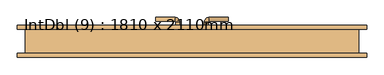
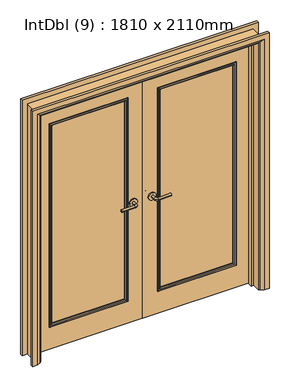
"""IFC4 building model written with IfcOpenShell, lengths in millimetres: door geometry, IntDbl (9) : 1810 x 2110mm."""

from ifc_helpers import new_model, si_unit, point, frame, frame_2d, origin, place, context, project, spatial, polyline, circle_curve, ellipse_curve, trimmed, segment, composite_curve, outline, extrude, faceted_brep, source, transform, mapped, element, save
from ifc_brep_helpers import plane_surface, cylinder_surface, revolved_surface, advanced_brep


def intdbl_9_1810_x_2110mm_150ef72f(model_context):
    return source(origin(), model_context, "Body", "SolidModel", [
        advanced_brep(
        [(-66.5, 25.0, 1007.0), (-86.5, 25.0, 1007.0), (-66.5, -5.0, 1007.0), (-86.5, -5.0, 1007.0), (-91.5, -10.0, 1007.0), (-91.5, -30.0, 1007.0), (-196.5, -30.0, 1007.0), (-196.5, -10.0, 1007.0)],
        [
            (0, 1, circle_curve(frame((-76.5, 25.0, 1007.0), z_axis=(0.0, 1.0, 0.0), x_axis=(-1.0, 0.0, 0.0)), 10.0)),
            (1, 0, circle_curve(frame((-76.5, 25.0, 1007.0), z_axis=(0.0, 1.0, 0.0), x_axis=(-1.0, 0.0, 0.0)), 10.0)),
            (0, 2),
            (2, 3, circle_curve(frame((-76.5, -5.0, 1007.0), z_axis=(0.0, 1.0, 0.0), x_axis=(-1.0, 0.0, 0.0)), 10.0)),
            (3, 1),
            (3, 2, circle_curve(frame((-76.5, -5.0, 1007.0), z_axis=(0.0, 1.0, 0.0), x_axis=(-1.0, 0.0, 0.0)), 10.0)),
            (4, 3, circle_curve(frame((-91.5, -5.0, 1007.0), z_axis=(0.0, 0.0, 1.0), x_axis=(1.0, 0.0, 0.0)), 5.0)),
            (2, 5, circle_curve(frame((-91.5, -5.0, 1007.0), z_axis=(0.0, 0.0, -1.0), x_axis=(1.0, 0.0, 0.0)), 25.0)),
            (5, 4, circle_curve(frame((-91.5, -20.0, 1007.0), z_axis=(1.0, 0.0, 0.0), x_axis=(0.0, 1.0, 0.0)), 10.0)),
            (4, 5, circle_curve(frame((-91.5, -20.0, 1007.0), z_axis=(1.0, 0.0, 0.0), x_axis=(0.0, 1.0, 0.0)), 10.0)),
            (6, 7, circle_curve(frame((-196.5, -20.0, 1007.0), z_axis=(-1.0, 0.0, 0.0), x_axis=(0.0, 1.0, 0.0)), 10.0)),
            (7, 6, circle_curve(frame((-196.5, -20.0, 1007.0), z_axis=(-1.0, 0.0, 0.0), x_axis=(0.0, 1.0, 0.0)), 10.0)),
            (5, 6),
            (7, 4),
        ],
        [
            plane_surface(frame((-76.5, 25.0, 1007.0), z_axis=(0.0, 1.0, 0.0), x_axis=(0.0, 0.0, 1.0))),
            cylinder_surface(frame((-76.5, 25.0, 1007.0), z_axis=(0.0, 1.0, 0.0), x_axis=(-1.0, 0.0, 0.0)), 10.0),
            revolved_surface(trimmed(ellipse_curve(frame((-76.5, -5.0, 1007.0), z_axis=(0.0, 1.0, 0.0), x_axis=(-1.0, 0.0, 0.0)), 10.0, 10.0), [point((-66.5, -5.0, 1007.0))], [point((-86.5, -5.0, 1007.0))], True, "CARTESIAN"), (-91.5, -5.0, 1007.0), (0.0, 0.0, -1.0)),
            revolved_surface(trimmed(ellipse_curve(frame((-76.5, -5.0, 1007.0), z_axis=(0.0, 1.0, 0.0), x_axis=(-1.0, 0.0, 0.0)), 10.0, 10.0), [point((-86.5, -5.0, 1007.0))], [point((-66.5, -5.0, 1007.0))], True, "CARTESIAN"), (-91.5, -5.0, 1007.0), (0.0, 0.0, -1.0)),
            plane_surface(frame((-196.5, -20.0, 1007.0), z_axis=(-1.0, 0.0, 0.0), x_axis=(0.0, 0.0, 1.0))),
            cylinder_surface(frame((-91.5, -20.0, 1007.0), z_axis=(1.0, 0.0, 0.0), x_axis=(0.0, 1.0, 0.0)), 10.0),
        ],
        [
            (0, [[1, 2]]),
            (1, [[-1, 3, 4, 5]]),
            (1, [[-2, -5, 6, -3]]),
            (2, [[7, -4, 8, 9]]),
            (3, [[-8, -6, -7, 10]]),
            (4, [[11, 12]]),
            (5, [[-9, 13, -12, 14]]),
            (5, [[-10, -14, -11, -13]]),
        ],
    ),
        extrude(outline(composite_curve([segment(trimmed(circle_curve(frame_2d((1007.0, -74.0)), 30.0), [point((1007.0, -44.0))], [point((1007.0, -104.0))], False, "CARTESIAN"), True, "CONTINUOUS"), segment(trimmed(circle_curve(frame_2d((1007.0, -74.0)), 30.0), [point((1007.0, -104.0))], [point((1007.0, -44.0))], False, "CARTESIAN"), True, "CONTINUOUS")], self_intersect=False)), frame((0.0, 25.0, 0.0), z_axis=(0.0, 1.0, 0.0), x_axis=(0.0, 0.0, 1.0)), (0.0, 0.0, 1.0), 8.0),
        advanced_brep(
        [(-66.5, 73.0, 1007.0), (-86.5, 73.0, 1007.0), (-86.5, 103.0, 1007.0), (-66.5, 103.0, 1007.0), (-91.5, 108.0, 1007.0), (-91.5, 128.0, 1007.0), (-196.5, 128.0, 1007.0), (-196.5, 108.0, 1007.0)],
        [
            (0, 1, circle_curve(frame((-76.5, 73.0, 1007.0), z_axis=(0.0, -1.0, 0.0), x_axis=(-1.0, 0.0, 0.0)), 10.0)),
            (1, 0, circle_curve(frame((-76.5, 73.0, 1007.0), z_axis=(0.0, -1.0, 0.0), x_axis=(-1.0, 0.0, 0.0)), 10.0)),
            (1, 2),
            (2, 3, circle_curve(frame((-76.5, 103.0, 1007.0), z_axis=(0.0, -1.0, 0.0), x_axis=(-1.0, 0.0, 0.0)), 10.0)),
            (3, 0),
            (3, 2, circle_curve(frame((-76.5, 103.0, 1007.0), z_axis=(0.0, -1.0, 0.0), x_axis=(-1.0, 0.0, 0.0)), 10.0)),
            (4, 5, circle_curve(frame((-91.5, 118.0, 1007.0), z_axis=(1.0, 0.0, 0.0), x_axis=(0.0, -1.0, 0.0)), 10.0)),
            (5, 3, circle_curve(frame((-91.5, 103.0, 1007.0), z_axis=(0.0, 0.0, -1.0), x_axis=(1.0, 0.0, 0.0)), 25.0)),
            (2, 4, circle_curve(frame((-91.5, 103.0, 1007.0), z_axis=(0.0, 0.0, 1.0), x_axis=(1.0, 0.0, 0.0)), 5.0)),
            (5, 4, circle_curve(frame((-91.5, 118.0, 1007.0), z_axis=(1.0, 0.0, 0.0), x_axis=(0.0, -1.0, 0.0)), 10.0)),
            (6, 7, circle_curve(frame((-196.5, 118.0, 1007.0), z_axis=(-1.0, 0.0, 0.0), x_axis=(0.0, -1.0, 0.0)), 10.0)),
            (7, 6, circle_curve(frame((-196.5, 118.0, 1007.0), z_axis=(-1.0, 0.0, 0.0), x_axis=(0.0, -1.0, 0.0)), 10.0)),
            (4, 7),
            (6, 5),
        ],
        [
            plane_surface(frame((-76.5, 73.0, 1007.0), z_axis=(0.0, -1.0, 0.0), x_axis=(0.0, 0.0, 1.0))),
            cylinder_surface(frame((-76.5, 73.0, 1007.0), z_axis=(0.0, -1.0, 0.0), x_axis=(-1.0, 0.0, 0.0)), 10.0),
            revolved_surface(trimmed(ellipse_curve(frame((-76.5, 103.0, 1007.0), z_axis=(0.0, 1.0, 0.0), x_axis=(-1.0, 0.0, 0.0)), 10.0, 10.0), [point((-66.5, 103.0, 1007.0))], [point((-86.5, 103.0, 1007.0))], True, "CARTESIAN"), (-91.5, 103.0, 1007.0), (0.0, 0.0, -1.0)),
            revolved_surface(trimmed(ellipse_curve(frame((-76.5, 103.0, 1007.0), z_axis=(0.0, 1.0, 0.0), x_axis=(-1.0, 0.0, 0.0)), 10.0, 10.0), [point((-86.5, 103.0, 1007.0))], [point((-66.5, 103.0, 1007.0))], True, "CARTESIAN"), (-91.5, 103.0, 1007.0), (0.0, 0.0, -1.0)),
            plane_surface(frame((-196.5, 118.0, 1007.0), z_axis=(-1.0, 0.0, 0.0), x_axis=(0.0, 0.0, 1.0))),
            cylinder_surface(frame((-91.5, 118.0, 1007.0), z_axis=(1.0, 0.0, 0.0), x_axis=(0.0, -1.0, 0.0)), 10.0),
        ],
        [
            (0, [[1, 2]]),
            (1, [[3, 4, 5, -2]]),
            (1, [[-5, 6, -3, -1]]),
            (2, [[7, 8, -4, 9]]),
            (3, [[10, -9, -6, -8]]),
            (4, [[11, 12]]),
            (5, [[13, -11, 14, -7]]),
            (5, [[-14, -12, -13, -10]]),
        ],
    ),
        extrude(outline(composite_curve([segment(trimmed(circle_curve(frame_2d((1007.0, -74.0)), 30.0), [point((1007.0, -44.0))], [point((1007.0, -104.0))], False, "CARTESIAN"), True, "CONTINUOUS"), segment(trimmed(circle_curve(frame_2d((1007.0, -74.0)), 30.0), [point((1007.0, -104.0))], [point((1007.0, -44.0))], False, "CARTESIAN"), True, "CONTINUOUS")], self_intersect=False)), frame((0.0, 65.0, 0.0), z_axis=(0.0, 1.0, 0.0), x_axis=(0.0, 0.0, 1.0)), (0.0, 0.0, 1.0), 8.0),
        advanced_brep(
        [(66.5, 25.0, 1007.0), (86.5, 25.0, 1007.0), (86.5, -5.0, 1007.0), (66.5, -5.0, 1007.0), (91.5, -10.0, 1007.0), (91.5, -30.0, 1007.0), (196.5, -30.0, 1007.0), (196.5, -10.0, 1007.0)],
        [
            (0, 1, circle_curve(frame((76.5, 25.0, 1007.0), z_axis=(0.0, 1.0, 0.0), x_axis=(1.0, 0.0, 0.0)), 10.0)),
            (1, 0, circle_curve(frame((76.5, 25.0, 1007.0), z_axis=(0.0, 1.0, 0.0), x_axis=(1.0, 0.0, 0.0)), 10.0)),
            (1, 2),
            (2, 3, circle_curve(frame((76.5, -5.0, 1007.0), z_axis=(0.0, 1.0, 0.0), x_axis=(1.0, 0.0, 0.0)), 10.0)),
            (3, 0),
            (3, 2, circle_curve(frame((76.5, -5.0, 1007.0), z_axis=(0.0, 1.0, 0.0), x_axis=(1.0, 0.0, 0.0)), 10.0)),
            (4, 5, circle_curve(frame((91.5, -20.0, 1007.0), z_axis=(-1.0, 0.0, 0.0), x_axis=(0.0, 1.0, 0.0)), 10.0)),
            (5, 3, circle_curve(frame((91.5, -5.0, 1007.0), z_axis=(0.0, 0.0, -1.0), x_axis=(-1.0, 0.0, 0.0)), 25.0)),
            (2, 4, circle_curve(frame((91.5, -5.0, 1007.0), z_axis=(0.0, 0.0, 1.0), x_axis=(-1.0, 0.0, 0.0)), 5.0)),
            (5, 4, circle_curve(frame((91.5, -20.0, 1007.0), z_axis=(-1.0, 0.0, 0.0), x_axis=(0.0, 1.0, 0.0)), 10.0)),
            (6, 7, circle_curve(frame((196.5, -20.0, 1007.0), z_axis=(1.0, 0.0, 0.0), x_axis=(0.0, 1.0, 0.0)), 10.0)),
            (7, 6, circle_curve(frame((196.5, -20.0, 1007.0), z_axis=(1.0, 0.0, 0.0), x_axis=(0.0, 1.0, 0.0)), 10.0)),
            (4, 7),
            (6, 5),
        ],
        [
            plane_surface(frame((76.5, 25.0, 1007.0), z_axis=(0.0, 1.0, 0.0), x_axis=(0.0, 0.0, 1.0))),
            cylinder_surface(frame((76.5, 25.0, 1007.0), z_axis=(0.0, 1.0, 0.0), x_axis=(1.0, 0.0, 0.0)), 10.0),
            revolved_surface(trimmed(ellipse_curve(frame((76.5, -5.0, 1007.0), z_axis=(0.0, -1.0, 0.0), x_axis=(1.0, 0.0, 0.0)), 10.0, 10.0), [point((66.5, -5.0, 1007.0))], [point((86.5, -5.0, 1007.0))], True, "CARTESIAN"), (91.5, -5.0, 1007.0), (0.0, 0.0, -1.0)),
            revolved_surface(trimmed(ellipse_curve(frame((76.5, -5.0, 1007.0), z_axis=(0.0, -1.0, 0.0), x_axis=(1.0, 0.0, 0.0)), 10.0, 10.0), [point((86.5, -5.0, 1007.0))], [point((66.5, -5.0, 1007.0))], True, "CARTESIAN"), (91.5, -5.0, 1007.0), (0.0, 0.0, -1.0)),
            plane_surface(frame((196.5, -20.0, 1007.0), z_axis=(1.0, 0.0, 0.0), x_axis=(0.0, 0.0, 1.0))),
            cylinder_surface(frame((91.5, -20.0, 1007.0), z_axis=(-1.0, 0.0, 0.0), x_axis=(0.0, 1.0, 0.0)), 10.0),
        ],
        [
            (0, [[1, 2]]),
            (1, [[3, 4, 5, -2]]),
            (1, [[-5, 6, -3, -1]]),
            (2, [[7, 8, -4, 9]]),
            (3, [[10, -9, -6, -8]]),
            (4, [[11, 12]]),
            (5, [[13, -11, 14, -7]]),
            (5, [[-14, -12, -13, -10]]),
        ],
    ),
        extrude(outline(composite_curve([segment(trimmed(circle_curve(frame_2d((1007.0, 74.0)), 30.0), [point((1007.0, 44.0))], [point((1007.0, 104.0))], False, "CARTESIAN"), True, "CONTINUOUS"), segment(trimmed(circle_curve(frame_2d((1007.0, 74.0)), 30.0), [point((1007.0, 104.0))], [point((1007.0, 44.0))], False, "CARTESIAN"), True, "CONTINUOUS")], self_intersect=False)), frame((0.0, 25.0, 0.0), z_axis=(0.0, 1.0, 0.0), x_axis=(0.0, 0.0, 1.0)), (0.0, 0.0, 1.0), 8.0),
        advanced_brep(
        [(66.5, 73.0, 1007.0), (86.5, 73.0, 1007.0), (66.5, 103.0, 1007.0), (86.5, 103.0, 1007.0), (91.5, 108.0, 1007.0), (91.5, 128.0, 1007.0), (196.5, 128.0, 1007.0), (196.5, 108.0, 1007.0)],
        [
            (0, 1, circle_curve(frame((76.5, 73.0, 1007.0), z_axis=(0.0, -1.0, 0.0), x_axis=(1.0, 0.0, 0.0)), 10.0)),
            (1, 0, circle_curve(frame((76.5, 73.0, 1007.0), z_axis=(0.0, -1.0, 0.0), x_axis=(1.0, 0.0, 0.0)), 10.0)),
            (0, 2),
            (2, 3, circle_curve(frame((76.5, 103.0, 1007.0), z_axis=(0.0, -1.0, 0.0), x_axis=(1.0, 0.0, 0.0)), 10.0)),
            (3, 1),
            (3, 2, circle_curve(frame((76.5, 103.0, 1007.0), z_axis=(0.0, -1.0, 0.0), x_axis=(1.0, 0.0, 0.0)), 10.0)),
            (4, 3, circle_curve(frame((91.5, 103.0, 1007.0), z_axis=(0.0, 0.0, 1.0), x_axis=(-1.0, 0.0, 0.0)), 5.0)),
            (2, 5, circle_curve(frame((91.5, 103.0, 1007.0), z_axis=(0.0, 0.0, -1.0), x_axis=(-1.0, 0.0, 0.0)), 25.0)),
            (5, 4, circle_curve(frame((91.5, 118.0, 1007.0), z_axis=(-1.0, 0.0, 0.0), x_axis=(0.0, -1.0, 0.0)), 10.0)),
            (4, 5, circle_curve(frame((91.5, 118.0, 1007.0), z_axis=(-1.0, 0.0, 0.0), x_axis=(0.0, -1.0, 0.0)), 10.0)),
            (6, 7, circle_curve(frame((196.5, 118.0, 1007.0), z_axis=(1.0, 0.0, 0.0), x_axis=(0.0, -1.0, 0.0)), 10.0)),
            (7, 6, circle_curve(frame((196.5, 118.0, 1007.0), z_axis=(1.0, 0.0, 0.0), x_axis=(0.0, -1.0, 0.0)), 10.0)),
            (5, 6),
            (7, 4),
        ],
        [
            plane_surface(frame((76.5, 73.0, 1007.0), z_axis=(0.0, -1.0, 0.0), x_axis=(0.0, 0.0, 1.0))),
            cylinder_surface(frame((76.5, 73.0, 1007.0), z_axis=(0.0, -1.0, 0.0), x_axis=(1.0, 0.0, 0.0)), 10.0),
            revolved_surface(trimmed(ellipse_curve(frame((76.5, 103.0, 1007.0), z_axis=(0.0, -1.0, 0.0), x_axis=(1.0, 0.0, 0.0)), 10.0, 10.0), [point((66.5, 103.0, 1007.0))], [point((86.5, 103.0, 1007.0))], True, "CARTESIAN"), (91.5, 103.0, 1007.0), (0.0, 0.0, -1.0)),
            revolved_surface(trimmed(ellipse_curve(frame((76.5, 103.0, 1007.0), z_axis=(0.0, -1.0, 0.0), x_axis=(1.0, 0.0, 0.0)), 10.0, 10.0), [point((86.5, 103.0, 1007.0))], [point((66.5, 103.0, 1007.0))], True, "CARTESIAN"), (91.5, 103.0, 1007.0), (0.0, 0.0, -1.0)),
            plane_surface(frame((196.5, 118.0, 1007.0), z_axis=(1.0, 0.0, 0.0), x_axis=(0.0, 0.0, 1.0))),
            cylinder_surface(frame((91.5, 118.0, 1007.0), z_axis=(-1.0, 0.0, 0.0), x_axis=(0.0, -1.0, 0.0)), 10.0),
        ],
        [
            (0, [[1, 2]]),
            (1, [[-1, 3, 4, 5]]),
            (1, [[-2, -5, 6, -3]]),
            (2, [[7, -4, 8, 9]]),
            (3, [[-8, -6, -7, 10]]),
            (4, [[11, 12]]),
            (5, [[-9, 13, -12, 14]]),
            (5, [[-10, -14, -11, -13]]),
        ],
    ),
        extrude(outline(composite_curve([segment(trimmed(circle_curve(frame_2d((1007.0, 74.0)), 30.0), [point((1007.0, 44.0))], [point((1007.0, 104.0))], False, "CARTESIAN"), True, "CONTINUOUS"), segment(trimmed(circle_curve(frame_2d((1007.0, 74.0)), 30.0), [point((1007.0, 104.0))], [point((1007.0, 44.0))], False, "CARTESIAN"), True, "CONTINUOUS")], self_intersect=False)), frame((0.0, 65.0, 0.0), z_axis=(0.0, 1.0, 0.0), x_axis=(0.0, 0.0, 1.0)), (0.0, 0.0, 1.0), 8.0),
        advanced_brep(
        [(-940.0, -85.0, 0.0), (-940.0, -65.0, 0.0), (-870.0, -65.0, 0.0), (-874.0, -71.0, 0.0), (-900.0, -85.0, 0.0), (-940.0, -85.0, 2145.0), (-940.0, -65.0, 2145.0), (940.0, -65.0, 2145.0), (940.0, -65.0, 0.0), (870.0, -65.0, 0.0), (870.0, -65.0, 2075.0), (-870.0, -65.0, 2075.0), (-874.0, -71.0, 2079.0), (-900.0, -85.0, 2105.0), (900.0, -85.0, 2105.0), (900.0, -85.0, 0.0), (940.0, -85.0, 0.0), (940.0, -85.0, 2145.0), (874.0, -71.0, 0.0), (874.0, -71.0, 2079.0)],
        [
            (0, 1),
            (1, 2),
            (2, 3, circle_curve(frame((-878.0, -64.0, 0.0), z_axis=(0.0, 0.0, -1.0), x_axis=(-1.0, 0.0, 0.0)), 8.0622577)),
            (3, 4),
            (4, 0),
            (0, 5),
            (5, 6),
            (6, 1),
            (6, 7),
            (7, 8),
            (8, 9),
            (9, 10),
            (10, 11),
            (11, 2),
            (11, 12, ellipse_curve(frame((-878.0, -64.0, 2083.0), z_axis=(-0.7071067811865475, 0.0, -0.7071067811865475), x_axis=(0.7071067811865474, 0.0, -0.7071067811865476)), 11.4017543, 8.0622577)),
            (12, 3),
            (12, 13),
            (13, 4),
            (13, 14),
            (14, 15),
            (15, 16),
            (16, 17),
            (17, 5),
            (7, 17),
            (16, 8),
            (15, 18),
            (18, 9, circle_curve(frame((878.0, -64.0, 0.0), z_axis=(0.0, 0.0, -1.0), x_axis=(1.0, 0.0, 0.0)), 8.0622577)),
            (19, 10, ellipse_curve(frame((878.0, -64.0, 2083.0), z_axis=(0.7071067811865475, 0.0, -0.7071067811865475), x_axis=(0.7071067811865474, 0.0, 0.7071067811865476)), 11.4017543, 8.0622577)),
            (18, 19),
            (14, 19),
            (19, 12),
        ],
        [
            plane_surface(frame((-870.0, -65.0, 0.0), z_axis=(0.0, 0.0, -1.0), x_axis=(0.0, -1.0, 0.0))),
            plane_surface(frame((-940.0, -85.0, 0.0), z_axis=(-1.0, 0.0, 0.0), x_axis=(0.0, 0.0, 1.0))),
            plane_surface(frame((-940.0, -65.0, 0.0), z_axis=(0.0, 1.0, 0.0), x_axis=(0.0, 0.0, 1.0))),
            cylinder_surface(frame((-878.0, -64.0, 0.0), z_axis=(0.0, 0.0, -1.0), x_axis=(-1.0, 0.0, 0.0)), 8.0622577),
            plane_surface(frame((-874.0, -71.0, 0.0), z_axis=(0.4740998230350183, -0.8804710999221749, 0.0), x_axis=(0.0, 0.0, 1.0))),
            plane_surface(frame((-900.0, -85.0, 0.0), z_axis=(0.0, -1.0, 0.0), x_axis=(0.0, 0.0, 1.0))),
            plane_surface(frame((940.0, -85.0, 2145.0), z_axis=(1.0, 0.0, 0.0), x_axis=(0.0, 0.0, -1.0))),
            plane_surface(frame((870.0, -65.0, 0.0), z_axis=(0.0, 0.0, -1.0), x_axis=(0.0, -1.0, 0.0))),
            cylinder_surface(frame((878.0, -64.0, 2075.0), z_axis=(0.0, 0.0, 1.0), x_axis=(1.0, 0.0, 0.0)), 8.0622577),
            plane_surface(frame((874.0, -71.0, 2079.0), z_axis=(-0.4740998230350183, -0.8804710999221749, 0.0), x_axis=(0.0, 0.0, -1.0))),
            plane_surface(frame((-940.0, -85.0, 2145.0), z_axis=(0.0, 0.0, 1.0), x_axis=(1.0, 0.0, 0.0))),
            cylinder_surface(frame((-870.0, -64.0, 2083.0), z_axis=(-1.0, 0.0, 0.0), x_axis=(0.0, 0.0, 1.0)), 8.0622577),
            plane_surface(frame((-874.0, -71.0, 2079.0), z_axis=(0.0, -0.8804710999221749, -0.4740998230350183), x_axis=(1.0, 0.0, 0.0))),
        ],
        [
            (0, [[1, 2, 3, 4, 5]]),
            (1, [[-1, 6, 7, 8]]),
            (2, [[-2, -8, 9, 10, 11, 12, 13, 14]]),
            (3, [[-3, -14, 15, 16]]),
            (4, [[-4, -16, 17, 18]]),
            (5, [[-5, -18, 19, 20, 21, 22, 23, -6]]),
            (6, [[24, -22, 25, -10]]),
            (7, [[-21, 26, 27, -11, -25]]),
            (8, [[28, -12, -27, 29]]),
            (9, [[30, -29, -26, -20]]),
            (10, [[-7, -23, -24, -9]]),
            (11, [[-15, -13, -28, 31]]),
            (12, [[-17, -31, -30, -19]]),
        ],
    ),
        advanced_brep(
        [(940.0, 85.0, 0.0), (940.0, 65.0, 0.0), (870.0, 65.0, 0.0), (874.0, 71.0, 0.0), (900.0, 85.0, 0.0), (940.0, 85.0, 2145.0), (940.0, 65.0, 2145.0), (-940.0, 65.0, 2145.0), (-940.0, 65.0, 0.0), (-870.0, 65.0, 0.0), (-870.0, 65.0, 2075.0), (870.0, 65.0, 2075.0), (874.0, 71.0, 2079.0), (900.0, 85.0, 2105.0), (-900.0, 85.0, 2105.0), (-900.0, 85.0, 0.0), (-940.0, 85.0, 0.0), (-940.0, 85.0, 2145.0), (-874.0, 71.0, 0.0), (-874.0, 71.0, 2079.0)],
        [
            (0, 1),
            (1, 2),
            (2, 3, circle_curve(frame((878.0, 64.0, 0.0), z_axis=(0.0, 0.0, -1.0), x_axis=(1.0, 0.0, 0.0)), 8.0622577)),
            (3, 4),
            (4, 0),
            (0, 5),
            (5, 6),
            (6, 1),
            (6, 7),
            (7, 8),
            (8, 9),
            (9, 10),
            (10, 11),
            (11, 2),
            (11, 12, ellipse_curve(frame((878.0, 64.0, 2083.0), z_axis=(0.7071067811865475, 0.0, -0.7071067811865475), x_axis=(-0.7071067811865474, 0.0, -0.7071067811865476)), 11.4017543, 8.0622577)),
            (12, 3),
            (12, 13),
            (13, 4),
            (13, 14),
            (14, 15),
            (15, 16),
            (16, 17),
            (17, 5),
            (7, 17),
            (16, 8),
            (15, 18),
            (18, 9, circle_curve(frame((-878.0, 64.0, 0.0), z_axis=(0.0, 0.0, -1.0), x_axis=(-1.0, 0.0, 0.0)), 8.0622577)),
            (19, 10, ellipse_curve(frame((-878.0, 64.0, 2083.0), z_axis=(-0.7071067811865475, 0.0, -0.7071067811865475), x_axis=(-0.7071067811865474, 0.0, 0.7071067811865476)), 11.4017543, 8.0622577)),
            (18, 19),
            (14, 19),
            (19, 12),
        ],
        [
            plane_surface(frame((870.0, 65.0, 0.0), z_axis=(0.0, 0.0, -1.0), x_axis=(0.0, -1.0, 0.0))),
            plane_surface(frame((940.0, 85.0, 0.0), z_axis=(1.0, 0.0, 0.0), x_axis=(0.0, 0.0, 1.0))),
            plane_surface(frame((940.0, 65.0, 0.0), z_axis=(0.0, -1.0, 0.0), x_axis=(0.0, 0.0, 1.0))),
            cylinder_surface(frame((878.0, 64.0, 0.0), z_axis=(0.0, 0.0, -1.0), x_axis=(1.0, 0.0, 0.0)), 8.0622577),
            plane_surface(frame((874.0, 71.0, 0.0), z_axis=(-0.4740998230350126, 0.8804710999221779, 0.0), x_axis=(0.0, 0.0, 1.0))),
            plane_surface(frame((900.0, 85.0, 0.0), z_axis=(0.0, 1.0, 0.0), x_axis=(0.0, 0.0, 1.0))),
            plane_surface(frame((-940.0, 85.0, 2145.0), z_axis=(-1.0, 0.0, 0.0), x_axis=(0.0, 0.0, -1.0))),
            plane_surface(frame((-870.0, 65.0, 0.0), z_axis=(0.0, 0.0, -1.0), x_axis=(0.0, -1.0, 0.0))),
            cylinder_surface(frame((-878.0, 64.0, 2075.0), z_axis=(0.0, 0.0, 1.0), x_axis=(-1.0, 0.0, 0.0)), 8.0622577),
            plane_surface(frame((-874.0, 71.0, 2079.0), z_axis=(0.4740998230350183, 0.8804710999221749, 0.0), x_axis=(0.0, 0.0, -1.0))),
            plane_surface(frame((940.0, 85.0, 2145.0), z_axis=(0.0, 0.0, 1.0), x_axis=(-1.0, 0.0, 0.0))),
            cylinder_surface(frame((870.0, 64.0, 2083.0), z_axis=(1.0, 0.0, 0.0), x_axis=(0.0, 0.0, 1.0)), 8.0622577),
            plane_surface(frame((874.0, 71.0, 2079.0), z_axis=(0.0, 0.8804710999221763, -0.4740998230350154), x_axis=(-1.0, 0.0, 0.0))),
        ],
        [
            (0, [[1, 2, 3, 4, 5]]),
            (1, [[-1, 6, 7, 8]]),
            (2, [[-2, -8, 9, 10, 11, 12, 13, 14]]),
            (3, [[-3, -14, 15, 16]]),
            (4, [[-4, -16, 17, 18]]),
            (5, [[-5, -18, 19, 20, 21, 22, 23, -6]]),
            (6, [[24, -22, 25, -10]]),
            (7, [[-21, 26, 27, -11, -25]]),
            (8, [[28, -12, -27, 29]]),
            (9, [[30, -29, -26, -20]]),
            (10, [[-7, -23, -24, -9]]),
            (11, [[-15, -13, -28, 31]]),
            (12, [[-17, -31, -30, -19]]),
        ],
    ),
        faceted_brep([(-846.0, 30.0, 0.0), (-846.0, -2.0, 0.0), (-865.0, -2.0, 0.0), (-865.0, 30.0, 0.0), (-846.0, 30.0, 2051.0), (-846.0, -2.0, 2051.0), (-865.0, -2.0, 2070.0), (-865.0, 30.0, 2070.0), (846.0, 30.0, 0.0), (865.0, 30.0, 0.0), (865.0, -2.0, 0.0), (846.0, -2.0, 0.0), (846.0, 30.0, 2051.0), (865.0, 30.0, 2070.0), (865.0, -2.0, 2070.0), (846.0, -2.0, 2051.0)], [[[0, 1, 2, 3]], [[1, 0, 4, 5]], [[2, 1, 5, 6]], [[3, 2, 6, 7]], [[0, 3, 7, 4]], [[8, 9, 10, 11]], [[12, 13, 9, 8]], [[13, 14, 10, 9]], [[14, 15, 11, 10]], [[15, 12, 8, 11]], [[5, 4, 12, 15]], [[6, 5, 15, 14]], [[7, 6, 14, 13]], [[4, 7, 13, 12]]]),
        extrude(outline(polyline([(2102.0, -897.0), (0.0, -897.0), (0.0, -865.0), (2070.0, -865.0), (2070.0, 865.0), (0.0, 865.0), (0.0, 897.0), (2102.0, 897.0), (2102.0, -897.0)])), frame((0.0, -65.0, 0.0), z_axis=(0.0, 1.0, 0.0), x_axis=(0.0, 0.0, 1.0)), (0.0, 0.0, 1.0), 130.0),
        extrude(outline(polyline([(-126.5, 43.0), (-737.0, 43.0), (-737.0, 55.0), (-126.5, 55.0), (-126.5, 43.0)])), frame((0.0, 0.0, 200.0), z_axis=(0.0, 0.0, 1.0), x_axis=(1.0, 0.0, 0.0)), (0.0, 0.0, 1.0), 1692.0),
        extrude(outline(polyline([(737.0, 43.0), (126.5, 43.0), (126.5, 55.0), (737.0, 55.0), (737.0, 43.0)])), frame((0.0, 0.0, 200.0), z_axis=(0.0, 0.0, 1.0), x_axis=(1.0, 0.0, 0.0)), (0.0, 0.0, 1.0), 1692.0),
        extrude(outline(polyline([(5.753223, -862.0), (5.753223, -1.5), (2067.0, -1.5), (2067.0, -862.0), (5.753223, -862.0)]), holes=[polyline([(1892.0, -737.0), (1892.0, -126.5), (200.0, -126.5), (200.0, -737.0), (1892.0, -737.0)])]), frame((0.0, 33.0, 0.0), z_axis=(0.0, 1.0, 0.0), x_axis=(0.0, 0.0, 1.0)), (0.0, 0.0, 1.0), 32.0),
        extrude(outline(polyline([(5.753223, 862.0), (2067.0, 862.0), (2067.0, 1.5), (5.753223, 1.5), (5.753223, 862.0)]), holes=[polyline([(1892.0, 126.5), (1892.0, 737.0), (200.0, 737.0), (200.0, 126.5), (1892.0, 126.5)])]), frame((0.0, 33.0, 0.0), z_axis=(0.0, 1.0, 0.0), x_axis=(0.0, 0.0, 1.0)), (0.0, 0.0, 1.0), 32.0),
        advanced_brep(
        [(-737.0, 55.0, 1892.0), (-737.0, 65.0, 1892.0), (-737.0, 65.0, 200.0), (-737.0, 55.0, 200.0), (-725.0, 66.0, 1880.0), (-725.0, 55.0, 1880.0), (-725.0, 55.0, 212.0), (-725.0, 66.0, 212.0), (-730.0, 71.0, 1885.0), (-730.0, 71.0, 207.0), (-745.0, 69.0, 1900.0), (-743.0, 71.0, 1898.0), (-743.0, 71.0, 194.0), (-745.0, 69.0, 192.0), (-745.0, 65.0, 1900.0), (-745.0, 65.0, 192.0), (-126.5, 65.0, 200.0), (-126.5, 55.0, 200.0), (-138.5, 55.0, 212.0), (-138.5, 66.0, 212.0), (-133.5, 71.0, 207.0), (-120.5, 71.0, 194.0), (-118.5, 69.0, 192.0), (-118.5, 65.0, 192.0), (-126.5, 65.0, 1892.0), (-126.5, 55.0, 1892.0), (-138.5, 55.0, 1880.0), (-138.5, 66.0, 1880.0), (-133.5, 71.0, 1885.0), (-120.5, 71.0, 1898.0), (-118.5, 69.0, 1900.0), (-118.5, 65.0, 1900.0)],
        [
            (0, 1),
            (1, 2),
            (2, 3),
            (3, 0),
            (4, 5),
            (5, 6),
            (6, 7),
            (7, 4),
            (8, 4, ellipse_curve(frame((-730.0, 66.0, 1885.0), z_axis=(-0.7071067811865475, 0.0, -0.7071067811865475), x_axis=(-0.7071067811865474, 0.0, 0.7071067811865476)), 7.0710678, 5.0)),
            (7, 9, ellipse_curve(frame((-730.0, 66.0, 207.0), z_axis=(-0.7071067811865475, 0.0, 0.7071067811865475), x_axis=(0.7071067811865474, 0.0, 0.7071067811865476)), 7.0710678, 5.0)),
            (9, 8),
            (10, 11, ellipse_curve(frame((-743.0, 69.0, 1898.0), z_axis=(-0.7071067811865475, 0.0, -0.7071067811865475), x_axis=(-0.7071067811865474, 0.0, 0.7071067811865476)), 2.8284271, 2.0)),
            (11, 12),
            (12, 13, ellipse_curve(frame((-743.0, 69.0, 194.0), z_axis=(-0.7071067811865475, 0.0, 0.7071067811865475), x_axis=(0.7071067811865474, 0.0, 0.7071067811865476)), 2.8284271, 2.0)),
            (13, 10),
            (14, 10),
            (13, 15),
            (15, 14),
            (2, 16),
            (16, 17),
            (17, 3),
            (6, 18),
            (18, 19),
            (19, 7),
            (19, 20, ellipse_curve(frame((-133.5, 66.0, 207.0), z_axis=(-0.7071067811865475, 0.0, -0.7071067811865475), x_axis=(-0.7071067811865476, 0.0, 0.7071067811865474)), 7.0710678, 5.0)),
            (20, 9),
            (12, 21),
            (21, 22, ellipse_curve(frame((-120.5, 69.0, 194.0), z_axis=(-0.7071067811865475, 0.0, -0.7071067811865475), x_axis=(-0.7071067811865476, 0.0, 0.7071067811865474)), 2.8284271, 2.0)),
            (22, 13),
            (22, 23),
            (23, 15),
            (16, 24),
            (24, 25),
            (25, 17),
            (18, 26),
            (26, 27),
            (27, 19),
            (27, 28, ellipse_curve(frame((-133.5, 66.0, 1885.0), z_axis=(0.7071067811865475, 0.0, -0.7071067811865475), x_axis=(-0.7071067811865474, 0.0, -0.7071067811865476)), 7.0710678, 5.0)),
            (28, 20),
            (21, 29),
            (29, 30, ellipse_curve(frame((-120.5, 69.0, 1898.0), z_axis=(0.7071067811865475, 0.0, -0.7071067811865475), x_axis=(-0.7071067811865474, 0.0, -0.7071067811865476)), 2.8284271, 2.0)),
            (30, 22),
            (30, 31),
            (31, 23),
            (31, 14),
            (1, 24),
            (0, 25),
            (5, 26),
            (4, 27),
            (8, 28),
            (11, 29),
            (10, 30),
        ],
        [
            plane_surface(frame((-737.0, 65.0, 1892.0), z_axis=(-1.0, 0.0, 0.0), x_axis=(0.0, 0.0, -1.0))),
            plane_surface(frame((-725.0, 55.0, 1880.0), z_axis=(1.0, 0.0, 0.0), x_axis=(0.0, 0.0, -1.0))),
            cylinder_surface(frame((-730.0, 66.0, 1892.0), z_axis=(0.0, 0.0, 1.0), x_axis=(-1.0, 0.0, 0.0)), 5.0),
            cylinder_surface(frame((-743.0, 69.0, 1892.0), z_axis=(0.0, 0.0, 1.0), x_axis=(-1.0, 0.0, 0.0)), 2.0),
            plane_surface(frame((-745.0, 69.0, 1900.0), z_axis=(-1.0, 0.0, 0.0), x_axis=(0.0, 0.0, -1.0))),
            plane_surface(frame((-737.0, 65.0, 200.0), z_axis=(0.0, 0.0, -1.0), x_axis=(1.0, 0.0, 0.0))),
            plane_surface(frame((-725.0, 55.0, 212.0), z_axis=(0.0, 0.0, 1.0), x_axis=(1.0, 0.0, 0.0))),
            cylinder_surface(frame((-737.0, 66.0, 207.0), z_axis=(-1.0, 0.0, 0.0), x_axis=(0.0, 0.0, -1.0)), 5.0),
            cylinder_surface(frame((-737.0, 69.0, 194.0), z_axis=(-1.0, 0.0, 0.0), x_axis=(0.0, 0.0, -1.0)), 2.0),
            plane_surface(frame((-745.0, 69.0, 192.0), z_axis=(0.0, 0.0, -1.0), x_axis=(1.0, 0.0, 0.0))),
            plane_surface(frame((-126.5, 65.0, 200.0), z_axis=(1.0, 0.0, 0.0), x_axis=(0.0, 0.0, 1.0))),
            plane_surface(frame((-138.5, 55.0, 212.0), z_axis=(-1.0, 0.0, 0.0), x_axis=(0.0, 0.0, 1.0))),
            cylinder_surface(frame((-133.5, 66.0, 200.0), z_axis=(0.0, 0.0, -1.0), x_axis=(1.0, 0.0, 0.0)), 5.0),
            cylinder_surface(frame((-120.5, 69.0, 200.0), z_axis=(0.0, 0.0, -1.0), x_axis=(1.0, 0.0, 0.0)), 2.0),
            plane_surface(frame((-118.5, 69.0, 192.0), z_axis=(1.0, 0.0, 0.0), x_axis=(0.0, 0.0, 1.0))),
            plane_surface(frame((-118.5, 65.0, 1900.0), z_axis=(0.0, -1.0, 0.0), x_axis=(-1.0, 0.0, 0.0))),
            plane_surface(frame((-126.5, 65.0, 1892.0), z_axis=(0.0, 0.0, 1.0), x_axis=(-1.0, 0.0, 0.0))),
            plane_surface(frame((-126.5, 55.0, 1892.0), z_axis=(0.0, -1.0, 0.0), x_axis=(-1.0, 0.0, 0.0))),
            plane_surface(frame((-138.5, 55.0, 1880.0), z_axis=(0.0, 0.0, -1.0), x_axis=(-1.0, 0.0, 0.0))),
            cylinder_surface(frame((-126.5, 66.0, 1885.0), z_axis=(1.0, 0.0, 0.0), x_axis=(0.0, 0.0, 1.0)), 5.0),
            plane_surface(frame((-133.5, 71.0, 1885.0), z_axis=(0.0, 1.0, 0.0), x_axis=(-1.0, 0.0, 0.0))),
            cylinder_surface(frame((-126.5, 69.0, 1898.0), z_axis=(1.0, 0.0, 0.0), x_axis=(0.0, 0.0, 1.0)), 2.0),
            plane_surface(frame((-118.5, 69.0, 1900.0), z_axis=(0.0, 0.0, 1.0), x_axis=(-1.0, 0.0, 0.0))),
        ],
        [
            (0, [[1, 2, 3, 4]]),
            (1, [[5, 6, 7, 8]]),
            (2, [[9, -8, 10, 11]]),
            (3, [[12, 13, 14, 15]]),
            (4, [[16, -15, 17, 18]]),
            (5, [[-3, 19, 20, 21]]),
            (6, [[-7, 22, 23, 24]]),
            (7, [[-10, -24, 25, 26]]),
            (8, [[-14, 27, 28, 29]]),
            (9, [[-17, -29, 30, 31]]),
            (10, [[-20, 32, 33, 34]]),
            (11, [[-23, 35, 36, 37]]),
            (12, [[-25, -37, 38, 39]]),
            (13, [[-28, 40, 41, 42]]),
            (14, [[-30, -42, 43, 44]]),
            (15, [[-31, -44, 45, -18], [46, -32, -19, -2]]),
            (16, [[-33, -46, -1, 47]]),
            (17, [[-21, -34, -47, -4], [48, -35, -22, -6]]),
            (18, [[-36, -48, -5, 49]]),
            (19, [[-38, -49, -9, 50]]),
            (20, [[51, -40, -27, -13], [-26, -39, -50, -11]]),
            (21, [[-41, -51, -12, 52]]),
            (22, [[-43, -52, -16, -45]]),
        ],
    ),
        advanced_brep(
        [(737.0, 43.0, 1892.0), (737.0, 33.0, 1892.0), (737.0, 33.0, 200.0), (737.0, 43.0, 200.0), (725.0, 32.0, 1880.0), (725.0, 43.0, 1880.0), (725.0, 43.0, 212.0), (725.0, 32.0, 212.0), (730.0, 27.0, 1885.0), (730.0, 27.0, 207.0), (745.0, 29.0, 1900.0), (743.0, 27.0, 1898.0), (743.0, 27.0, 194.0), (745.0, 29.0, 192.0), (745.0, 33.0, 1900.0), (745.0, 33.0, 192.0), (126.5, 33.0, 200.0), (126.5, 43.0, 200.0), (138.5, 43.0, 212.0), (138.5, 32.0, 212.0), (133.5, 27.0, 207.0), (120.5, 27.0, 194.0), (118.5, 29.0, 192.0), (118.5, 33.0, 192.0), (126.5, 33.0, 1892.0), (126.5, 43.0, 1892.0), (138.5, 43.0, 1880.0), (138.5, 32.0, 1880.0), (133.5, 27.0, 1885.0), (120.5, 27.0, 1898.0), (118.5, 29.0, 1900.0), (118.5, 33.0, 1900.0)],
        [
            (0, 1),
            (1, 2),
            (2, 3),
            (3, 0),
            (4, 5),
            (5, 6),
            (6, 7),
            (7, 4),
            (8, 4, ellipse_curve(frame((730.0, 32.0, 1885.0), z_axis=(0.7071067811865475, 0.0, -0.7071067811865475), x_axis=(0.7071067811865474, 0.0, 0.7071067811865476)), 7.0710678, 5.0)),
            (7, 9, ellipse_curve(frame((730.0, 32.0, 207.0), z_axis=(0.7071067811865475, 0.0, 0.7071067811865475), x_axis=(-0.7071067811865474, 0.0, 0.7071067811865476)), 7.0710678, 5.0)),
            (9, 8),
            (10, 11, ellipse_curve(frame((743.0, 29.0, 1898.0), z_axis=(0.7071067811865475, 0.0, -0.7071067811865475), x_axis=(0.7071067811865474, 0.0, 0.7071067811865476)), 2.8284271, 2.0)),
            (11, 12),
            (12, 13, ellipse_curve(frame((743.0, 29.0, 194.0), z_axis=(0.7071067811865475, 0.0, 0.7071067811865475), x_axis=(-0.7071067811865474, 0.0, 0.7071067811865476)), 2.8284271, 2.0)),
            (13, 10),
            (14, 10),
            (13, 15),
            (15, 14),
            (2, 16),
            (16, 17),
            (17, 3),
            (6, 18),
            (18, 19),
            (19, 7),
            (19, 20, ellipse_curve(frame((133.5, 32.0, 207.0), z_axis=(0.7071067811865475, 0.0, -0.7071067811865475), x_axis=(0.7071067811865476, 0.0, 0.7071067811865474)), 7.0710678, 5.0)),
            (20, 9),
            (12, 21),
            (21, 22, ellipse_curve(frame((120.5, 29.0, 194.0), z_axis=(0.7071067811865475, 0.0, -0.7071067811865475), x_axis=(0.7071067811865476, 0.0, 0.7071067811865474)), 2.8284271, 2.0)),
            (22, 13),
            (22, 23),
            (23, 15),
            (16, 24),
            (24, 25),
            (25, 17),
            (18, 26),
            (26, 27),
            (27, 19),
            (27, 28, ellipse_curve(frame((133.5, 32.0, 1885.0), z_axis=(-0.7071067811865475, 0.0, -0.7071067811865475), x_axis=(0.7071067811865474, 0.0, -0.7071067811865476)), 7.0710678, 5.0)),
            (28, 20),
            (21, 29),
            (29, 30, ellipse_curve(frame((120.5, 29.0, 1898.0), z_axis=(-0.7071067811865475, 0.0, -0.7071067811865475), x_axis=(0.7071067811865474, 0.0, -0.7071067811865476)), 2.8284271, 2.0)),
            (30, 22),
            (30, 31),
            (31, 23),
            (31, 14),
            (1, 24),
            (0, 25),
            (5, 26),
            (4, 27),
            (8, 28),
            (11, 29),
            (10, 30),
        ],
        [
            plane_surface(frame((737.0, 33.0, 1892.0), z_axis=(1.0, 0.0, 0.0), x_axis=(0.0, 0.0, -1.0))),
            plane_surface(frame((725.0, 43.0, 1880.0), z_axis=(-1.0, 0.0, 0.0), x_axis=(0.0, 0.0, -1.0))),
            cylinder_surface(frame((730.0, 32.0, 1892.0), z_axis=(0.0, 0.0, 1.0), x_axis=(1.0, 0.0, 0.0)), 5.0),
            cylinder_surface(frame((743.0, 29.0, 1892.0), z_axis=(0.0, 0.0, 1.0), x_axis=(1.0, 0.0, 0.0)), 2.0),
            plane_surface(frame((745.0, 29.0, 1900.0), z_axis=(1.0, 0.0, 0.0), x_axis=(0.0, 0.0, -1.0))),
            plane_surface(frame((737.0, 33.0, 200.0), z_axis=(0.0, 0.0, -1.0), x_axis=(-1.0, 0.0, 0.0))),
            plane_surface(frame((725.0, 43.0, 212.0), z_axis=(0.0, 0.0, 1.0), x_axis=(-1.0, 0.0, 0.0))),
            cylinder_surface(frame((737.0, 32.0, 207.0), z_axis=(1.0, 0.0, 0.0), x_axis=(0.0, 0.0, -1.0)), 5.0),
            cylinder_surface(frame((737.0, 29.0, 194.0), z_axis=(1.0, 0.0, 0.0), x_axis=(0.0, 0.0, -1.0)), 2.0),
            plane_surface(frame((745.0, 29.0, 192.0), z_axis=(0.0, 0.0, -1.0), x_axis=(-1.0, 0.0, 0.0))),
            plane_surface(frame((126.5, 33.0, 200.0), z_axis=(-1.0, 0.0, 0.0), x_axis=(0.0, 0.0, 1.0))),
            plane_surface(frame((138.5, 43.0, 212.0), z_axis=(1.0, 0.0, 0.0), x_axis=(0.0, 0.0, 1.0))),
            cylinder_surface(frame((133.5, 32.0, 200.0), z_axis=(0.0, 0.0, -1.0), x_axis=(-1.0, 0.0, 0.0)), 5.0),
            cylinder_surface(frame((120.5, 29.0, 200.0), z_axis=(0.0, 0.0, -1.0), x_axis=(-1.0, 0.0, 0.0)), 2.0),
            plane_surface(frame((118.5, 29.0, 192.0), z_axis=(-1.0, 0.0, 0.0), x_axis=(0.0, 0.0, 1.0))),
            plane_surface(frame((118.5, 33.0, 1900.0), z_axis=(0.0, 1.0, 0.0), x_axis=(1.0, 0.0, 0.0))),
            plane_surface(frame((126.5, 33.0, 1892.0), z_axis=(0.0, 0.0, 1.0), x_axis=(1.0, 0.0, 0.0))),
            plane_surface(frame((126.5, 43.0, 1892.0), z_axis=(0.0, 1.0, 0.0), x_axis=(1.0, 0.0, 0.0))),
            plane_surface(frame((138.5, 43.0, 1880.0), z_axis=(0.0, 0.0, -1.0), x_axis=(1.0, 0.0, 0.0))),
            cylinder_surface(frame((126.5, 32.0, 1885.0), z_axis=(-1.0, 0.0, 0.0), x_axis=(0.0, 0.0, 1.0)), 5.0),
            plane_surface(frame((133.5, 27.0, 1885.0), z_axis=(0.0, -1.0, 0.0), x_axis=(1.0, 0.0, 0.0))),
            cylinder_surface(frame((126.5, 29.0, 1898.0), z_axis=(-1.0, 0.0, 0.0), x_axis=(0.0, 0.0, 1.0)), 2.0),
            plane_surface(frame((118.5, 29.0, 1900.0), z_axis=(0.0, 0.0, 1.0), x_axis=(1.0, 0.0, 0.0))),
        ],
        [
            (0, [[1, 2, 3, 4]]),
            (1, [[5, 6, 7, 8]]),
            (2, [[9, -8, 10, 11]]),
            (3, [[12, 13, 14, 15]]),
            (4, [[16, -15, 17, 18]]),
            (5, [[-3, 19, 20, 21]]),
            (6, [[-7, 22, 23, 24]]),
            (7, [[-10, -24, 25, 26]]),
            (8, [[-14, 27, 28, 29]]),
            (9, [[-17, -29, 30, 31]]),
            (10, [[-20, 32, 33, 34]]),
            (11, [[-23, 35, 36, 37]]),
            (12, [[-25, -37, 38, 39]]),
            (13, [[-28, 40, 41, 42]]),
            (14, [[-30, -42, 43, 44]]),
            (15, [[-31, -44, 45, -18], [46, -32, -19, -2]]),
            (16, [[-33, -46, -1, 47]]),
            (17, [[-21, -34, -47, -4], [48, -35, -22, -6]]),
            (18, [[-36, -48, -5, 49]]),
            (19, [[-38, -49, -9, 50]]),
            (20, [[51, -40, -27, -13], [-26, -39, -50, -11]]),
            (21, [[-41, -51, -12, 52]]),
            (22, [[-43, -52, -16, -45]]),
        ],
    ),
        advanced_brep(
        [(-126.5, 43.0, 1892.0), (-126.5, 33.0, 1892.0), (-126.5, 33.0, 200.0), (-126.5, 43.0, 200.0), (-138.5, 32.0, 1880.0), (-138.5, 43.0, 1880.0), (-138.5, 43.0, 212.0), (-138.5, 32.0, 212.0), (-133.5, 27.0, 1885.0), (-133.5, 27.0, 207.0), (-118.5, 29.0, 1900.0), (-120.5, 27.0, 1898.0), (-120.5, 27.0, 194.0), (-118.5, 29.0, 192.0), (-118.5, 33.0, 1900.0), (-118.5, 33.0, 192.0), (-737.0, 33.0, 200.0), (-737.0, 43.0, 200.0), (-725.0, 43.0, 212.0), (-725.0, 32.0, 212.0), (-730.0, 27.0, 207.0), (-743.0, 27.0, 194.0), (-745.0, 29.0, 192.0), (-745.0, 33.0, 192.0), (-737.0, 33.0, 1892.0), (-737.0, 43.0, 1892.0), (-725.0, 43.0, 1880.0), (-725.0, 32.0, 1880.0), (-730.0, 27.0, 1885.0), (-743.0, 27.0, 1898.0), (-745.0, 29.0, 1900.0), (-745.0, 33.0, 1900.0)],
        [
            (0, 1),
            (1, 2),
            (2, 3),
            (3, 0),
            (4, 5),
            (5, 6),
            (6, 7),
            (7, 4),
            (8, 4, ellipse_curve(frame((-133.5, 32.0, 1885.0), z_axis=(0.7071067811865475, 0.0, -0.7071067811865475), x_axis=(0.7071067811865474, 0.0, 0.7071067811865476)), 7.0710678, 5.0)),
            (7, 9, ellipse_curve(frame((-133.5, 32.0, 207.0), z_axis=(0.7071067811865475, 0.0, 0.7071067811865475), x_axis=(-0.7071067811865474, 0.0, 0.7071067811865476)), 7.0710678, 5.0)),
            (9, 8),
            (10, 11, ellipse_curve(frame((-120.5, 29.0, 1898.0), z_axis=(0.7071067811865475, 0.0, -0.7071067811865475), x_axis=(0.7071067811865474, 0.0, 0.7071067811865476)), 2.8284271, 2.0)),
            (11, 12),
            (12, 13, ellipse_curve(frame((-120.5, 29.0, 194.0), z_axis=(0.7071067811865475, 0.0, 0.7071067811865475), x_axis=(-0.7071067811865474, 0.0, 0.7071067811865476)), 2.8284271, 2.0)),
            (13, 10),
            (14, 10),
            (13, 15),
            (15, 14),
            (2, 16),
            (16, 17),
            (17, 3),
            (6, 18),
            (18, 19),
            (19, 7),
            (19, 20, ellipse_curve(frame((-730.0, 32.0, 207.0), z_axis=(0.7071067811865475, 0.0, -0.7071067811865475), x_axis=(0.7071067811865476, 0.0, 0.7071067811865474)), 7.0710678, 5.0)),
            (20, 9),
            (12, 21),
            (21, 22, ellipse_curve(frame((-743.0, 29.0, 194.0), z_axis=(0.7071067811865475, 0.0, -0.7071067811865475), x_axis=(0.7071067811865476, 0.0, 0.7071067811865474)), 2.8284271, 2.0)),
            (22, 13),
            (22, 23),
            (23, 15),
            (16, 24),
            (24, 25),
            (25, 17),
            (18, 26),
            (26, 27),
            (27, 19),
            (27, 28, ellipse_curve(frame((-730.0, 32.0, 1885.0), z_axis=(-0.7071067811865475, 0.0, -0.7071067811865475), x_axis=(0.7071067811865474, 0.0, -0.7071067811865476)), 7.0710678, 5.0)),
            (28, 20),
            (21, 29),
            (29, 30, ellipse_curve(frame((-743.0, 29.0, 1898.0), z_axis=(-0.7071067811865475, 0.0, -0.7071067811865475), x_axis=(0.7071067811865474, 0.0, -0.7071067811865476)), 2.8284271, 2.0)),
            (30, 22),
            (30, 31),
            (31, 23),
            (31, 14),
            (1, 24),
            (0, 25),
            (5, 26),
            (4, 27),
            (8, 28),
            (11, 29),
            (10, 30),
        ],
        [
            plane_surface(frame((-126.5, 33.0, 1892.0), z_axis=(1.0, 0.0, 0.0), x_axis=(0.0, 0.0, -1.0))),
            plane_surface(frame((-138.5, 43.0, 1880.0), z_axis=(-1.0, 0.0, 0.0), x_axis=(0.0, 0.0, -1.0))),
            cylinder_surface(frame((-133.5, 32.0, 1892.0), z_axis=(0.0, 0.0, 1.0), x_axis=(1.0, 0.0, 0.0)), 5.0),
            cylinder_surface(frame((-120.5, 29.0, 1892.0), z_axis=(0.0, 0.0, 1.0), x_axis=(1.0, 0.0, 0.0)), 2.0),
            plane_surface(frame((-118.5, 29.0, 1900.0), z_axis=(1.0, 0.0, 0.0), x_axis=(0.0, 0.0, -1.0))),
            plane_surface(frame((-126.5, 33.0, 200.0), z_axis=(0.0, 0.0, -1.0), x_axis=(-1.0, 0.0, 0.0))),
            plane_surface(frame((-138.5, 43.0, 212.0), z_axis=(0.0, 0.0, 1.0), x_axis=(-1.0, 0.0, 0.0))),
            cylinder_surface(frame((-126.5, 32.0, 207.0), z_axis=(1.0, 0.0, 0.0), x_axis=(0.0, 0.0, -1.0)), 5.0),
            cylinder_surface(frame((-126.5, 29.0, 194.0), z_axis=(1.0, 0.0, 0.0), x_axis=(0.0, 0.0, -1.0)), 2.0),
            plane_surface(frame((-118.5, 29.0, 192.0), z_axis=(0.0, 0.0, -1.0), x_axis=(-1.0, 0.0, 0.0))),
            plane_surface(frame((-737.0, 33.0, 200.0), z_axis=(-1.0, 0.0, 0.0), x_axis=(0.0, 0.0, 1.0))),
            plane_surface(frame((-725.0, 43.0, 212.0), z_axis=(1.0, 0.0, 0.0), x_axis=(0.0, 0.0, 1.0))),
            cylinder_surface(frame((-730.0, 32.0, 200.0), z_axis=(0.0, 0.0, -1.0), x_axis=(-1.0, 0.0, 0.0)), 5.0),
            cylinder_surface(frame((-743.0, 29.0, 200.0), z_axis=(0.0, 0.0, -1.0), x_axis=(-1.0, 0.0, 0.0)), 2.0),
            plane_surface(frame((-745.0, 29.0, 192.0), z_axis=(-1.0, 0.0, 0.0), x_axis=(0.0, 0.0, 1.0))),
            plane_surface(frame((-745.0, 33.0, 1900.0), z_axis=(0.0, 1.0, 0.0), x_axis=(1.0, 0.0, 0.0))),
            plane_surface(frame((-737.0, 33.0, 1892.0), z_axis=(0.0, 0.0, 1.0), x_axis=(1.0, 0.0, 0.0))),
            plane_surface(frame((-737.0, 43.0, 1892.0), z_axis=(0.0, 1.0, 0.0), x_axis=(1.0, 0.0, 0.0))),
            plane_surface(frame((-725.0, 43.0, 1880.0), z_axis=(0.0, 0.0, -1.0), x_axis=(1.0, 0.0, 0.0))),
            cylinder_surface(frame((-737.0, 32.0, 1885.0), z_axis=(-1.0, 0.0, 0.0), x_axis=(0.0, 0.0, 1.0)), 5.0),
            plane_surface(frame((-730.0, 27.0, 1885.0), z_axis=(0.0, -1.0, 0.0), x_axis=(1.0, 0.0, 0.0))),
            cylinder_surface(frame((-737.0, 29.0, 1898.0), z_axis=(-1.0, 0.0, 0.0), x_axis=(0.0, 0.0, 1.0)), 2.0),
            plane_surface(frame((-745.0, 29.0, 1900.0), z_axis=(0.0, 0.0, 1.0), x_axis=(1.0, 0.0, 0.0))),
        ],
        [
            (0, [[1, 2, 3, 4]]),
            (1, [[5, 6, 7, 8]]),
            (2, [[9, -8, 10, 11]]),
            (3, [[12, 13, 14, 15]]),
            (4, [[16, -15, 17, 18]]),
            (5, [[-3, 19, 20, 21]]),
            (6, [[-7, 22, 23, 24]]),
            (7, [[-10, -24, 25, 26]]),
            (8, [[-14, 27, 28, 29]]),
            (9, [[-17, -29, 30, 31]]),
            (10, [[-20, 32, 33, 34]]),
            (11, [[-23, 35, 36, 37]]),
            (12, [[-25, -37, 38, 39]]),
            (13, [[-28, 40, 41, 42]]),
            (14, [[-30, -42, 43, 44]]),
            (15, [[-31, -44, 45, -18], [46, -32, -19, -2]]),
            (16, [[-33, -46, -1, 47]]),
            (17, [[-21, -34, -47, -4], [48, -35, -22, -6]]),
            (18, [[-36, -48, -5, 49]]),
            (19, [[-38, -49, -9, 50]]),
            (20, [[51, -40, -27, -13], [-26, -39, -50, -11]]),
            (21, [[-41, -51, -12, 52]]),
            (22, [[-43, -52, -16, -45]]),
        ],
    ),
        advanced_brep(
        [(118.5, 69.0, 192.0), (118.5, 65.0, 192.0), (118.5, 65.0, 1900.0), (118.5, 69.0, 1900.0), (120.5, 71.0, 194.0), (120.5, 71.0, 1898.0), (138.5, 66.0, 212.0), (133.5, 71.0, 207.0), (133.5, 71.0, 1885.0), (138.5, 66.0, 1880.0), (138.5, 55.0, 212.0), (138.5, 55.0, 1880.0), (126.5, 65.0, 200.0), (126.5, 55.0, 200.0), (126.5, 55.0, 1892.0), (126.5, 65.0, 1892.0), (745.0, 65.0, 1900.0), (745.0, 69.0, 1900.0), (743.0, 71.0, 1898.0), (730.0, 71.0, 1885.0), (725.0, 66.0, 1880.0), (725.0, 55.0, 1880.0), (737.0, 55.0, 1892.0), (737.0, 65.0, 1892.0), (745.0, 65.0, 192.0), (745.0, 69.0, 192.0), (743.0, 71.0, 194.0), (730.0, 71.0, 207.0), (725.0, 66.0, 212.0), (725.0, 55.0, 212.0), (737.0, 55.0, 200.0), (737.0, 65.0, 200.0)],
        [
            (0, 1),
            (1, 2),
            (2, 3),
            (3, 0),
            (4, 0, ellipse_curve(frame((120.5, 69.0, 194.0), z_axis=(-0.7071067811865475, 0.0, 0.7071067811865475), x_axis=(-0.7071067811865474, 0.0, -0.7071067811865476)), 2.8284271, 2.0)),
            (3, 5, ellipse_curve(frame((120.5, 69.0, 1898.0), z_axis=(-0.7071067811865475, 0.0, -0.7071067811865475), x_axis=(0.7071067811865474, 0.0, -0.7071067811865476)), 2.8284271, 2.0)),
            (5, 4),
            (6, 7, ellipse_curve(frame((133.5, 66.0, 207.0), z_axis=(-0.7071067811865475, 0.0, 0.7071067811865475), x_axis=(-0.7071067811865474, 0.0, -0.7071067811865476)), 7.0710678, 5.0)),
            (7, 8),
            (8, 9, ellipse_curve(frame((133.5, 66.0, 1885.0), z_axis=(-0.7071067811865475, 0.0, -0.7071067811865475), x_axis=(0.7071067811865474, 0.0, -0.7071067811865476)), 7.0710678, 5.0)),
            (9, 6),
            (10, 6),
            (9, 11),
            (11, 10),
            (12, 13),
            (13, 14),
            (14, 15),
            (15, 12),
            (2, 16),
            (16, 17),
            (17, 3),
            (17, 18, ellipse_curve(frame((743.0, 69.0, 1898.0), z_axis=(-0.7071067811865475, 0.0, 0.7071067811865475), x_axis=(-0.7071067811865476, 0.0, -0.7071067811865474)), 2.8284271, 2.0)),
            (18, 5),
            (8, 19),
            (19, 20, ellipse_curve(frame((730.0, 66.0, 1885.0), z_axis=(-0.7071067811865475, 0.0, 0.7071067811865475), x_axis=(-0.7071067811865476, 0.0, -0.7071067811865474)), 7.0710678, 5.0)),
            (20, 9),
            (20, 21),
            (21, 11),
            (14, 22),
            (22, 23),
            (23, 15),
            (16, 24),
            (24, 25),
            (25, 17),
            (25, 26, ellipse_curve(frame((743.0, 69.0, 194.0), z_axis=(0.7071067811865475, 0.0, 0.7071067811865475), x_axis=(-0.7071067811865474, 0.0, 0.7071067811865476)), 2.8284271, 2.0)),
            (26, 18),
            (19, 27),
            (27, 28, ellipse_curve(frame((730.0, 66.0, 207.0), z_axis=(0.7071067811865475, 0.0, 0.7071067811865475), x_axis=(-0.7071067811865474, 0.0, 0.7071067811865476)), 7.0710678, 5.0)),
            (28, 20),
            (28, 29),
            (29, 21),
            (22, 30),
            (30, 31),
            (31, 23),
            (24, 1),
            (0, 25),
            (4, 26),
            (7, 27),
            (6, 28),
            (10, 29),
            (13, 30),
            (12, 31),
        ],
        [
            plane_surface(frame((118.5, 65.0, 192.0), z_axis=(-1.0, 0.0, 0.0), x_axis=(0.0, 0.0, 1.0))),
            cylinder_surface(frame((120.5, 69.0, 200.0), z_axis=(0.0, 0.0, -1.0), x_axis=(-1.0, 0.0, 0.0)), 2.0),
            cylinder_surface(frame((133.5, 66.0, 200.0), z_axis=(0.0, 0.0, -1.0), x_axis=(-1.0, 0.0, 0.0)), 5.0),
            plane_surface(frame((138.5, 66.0, 212.0), z_axis=(1.0, 0.0, 0.0), x_axis=(0.0, 0.0, 1.0))),
            plane_surface(frame((126.5, 55.0, 200.0), z_axis=(-1.0, 0.0, 0.0), x_axis=(0.0, 0.0, 1.0))),
            plane_surface(frame((118.5, 65.0, 1900.0), z_axis=(0.0, 0.0, 1.0), x_axis=(1.0, 0.0, 0.0))),
            cylinder_surface(frame((126.5, 69.0, 1898.0), z_axis=(-1.0, 0.0, 0.0), x_axis=(0.0, 0.0, 1.0)), 2.0),
            cylinder_surface(frame((126.5, 66.0, 1885.0), z_axis=(-1.0, 0.0, 0.0), x_axis=(0.0, 0.0, 1.0)), 5.0),
            plane_surface(frame((138.5, 66.0, 1880.0), z_axis=(0.0, 0.0, -1.0), x_axis=(1.0, 0.0, 0.0))),
            plane_surface(frame((126.5, 55.0, 1892.0), z_axis=(0.0, 0.0, 1.0), x_axis=(1.0, 0.0, 0.0))),
            plane_surface(frame((745.0, 65.0, 1900.0), z_axis=(1.0, 0.0, 0.0), x_axis=(0.0, 0.0, -1.0))),
            cylinder_surface(frame((743.0, 69.0, 1892.0), z_axis=(0.0, 0.0, 1.0), x_axis=(1.0, 0.0, 0.0)), 2.0),
            cylinder_surface(frame((730.0, 66.0, 1892.0), z_axis=(0.0, 0.0, 1.0), x_axis=(1.0, 0.0, 0.0)), 5.0),
            plane_surface(frame((725.0, 66.0, 1880.0), z_axis=(-1.0, 0.0, 0.0), x_axis=(0.0, 0.0, -1.0))),
            plane_surface(frame((737.0, 55.0, 1892.0), z_axis=(1.0, 0.0, 0.0), x_axis=(0.0, 0.0, -1.0))),
            plane_surface(frame((745.0, 65.0, 192.0), z_axis=(0.0, 0.0, -1.0), x_axis=(-1.0, 0.0, 0.0))),
            cylinder_surface(frame((737.0, 69.0, 194.0), z_axis=(1.0, 0.0, 0.0), x_axis=(0.0, 0.0, -1.0)), 2.0),
            plane_surface(frame((743.0, 71.0, 194.0), z_axis=(0.0, 1.0, 0.0), x_axis=(-1.0, 0.0, 0.0))),
            cylinder_surface(frame((737.0, 66.0, 207.0), z_axis=(1.0, 0.0, 0.0), x_axis=(0.0, 0.0, -1.0)), 5.0),
            plane_surface(frame((725.0, 66.0, 212.0), z_axis=(0.0, 0.0, 1.0), x_axis=(-1.0, 0.0, 0.0))),
            plane_surface(frame((725.0, 55.0, 212.0), z_axis=(0.0, -1.0, 0.0), x_axis=(-1.0, 0.0, 0.0))),
            plane_surface(frame((737.0, 55.0, 200.0), z_axis=(0.0, 0.0, -1.0), x_axis=(-1.0, 0.0, 0.0))),
            plane_surface(frame((737.0, 65.0, 200.0), z_axis=(0.0, -1.0, 0.0), x_axis=(-1.0, 0.0, 0.0))),
        ],
        [
            (0, [[1, 2, 3, 4]]),
            (1, [[5, -4, 6, 7]]),
            (2, [[8, 9, 10, 11]]),
            (3, [[12, -11, 13, 14]]),
            (4, [[15, 16, 17, 18]]),
            (5, [[-3, 19, 20, 21]]),
            (6, [[-6, -21, 22, 23]]),
            (7, [[-10, 24, 25, 26]]),
            (8, [[-13, -26, 27, 28]]),
            (9, [[-17, 29, 30, 31]]),
            (10, [[-20, 32, 33, 34]]),
            (11, [[-22, -34, 35, 36]]),
            (12, [[-25, 37, 38, 39]]),
            (13, [[-27, -39, 40, 41]]),
            (14, [[-30, 42, 43, 44]]),
            (15, [[-33, 45, -1, 46]]),
            (16, [[-35, -46, -5, 47]]),
            (17, [[-23, -36, -47, -7], [48, -37, -24, -9]]),
            (18, [[-38, -48, -8, 49]]),
            (19, [[-40, -49, -12, 50]]),
            (20, [[51, -42, -29, -16], [-28, -41, -50, -14]]),
            (21, [[-43, -51, -15, 52]]),
            (22, [[-45, -32, -19, -2], [-31, -44, -52, -18]]),
        ],
    ),
        extrude(outline(polyline([(200.0, 421.75), (200.0, 441.75), (528.4, 441.75), (528.4, 737.0), (548.4, 737.0), (548.4, 441.75), (866.8, 441.75), (866.8, 737.0), (886.8, 737.0), (886.8, 441.75), (1205.2, 441.75), (1205.2, 737.0), (1225.2, 737.0), (1225.2, 441.75), (1543.6, 441.75), (1543.6, 737.0), (1563.6, 737.0), (1563.6, 441.75), (1892.0, 441.75), (1892.0, 421.75), (1563.6, 421.75), (1563.6, 126.5), (1543.6, 126.5), (1543.6, 421.75), (1225.2, 421.75), (1225.2, 126.5), (1205.2, 126.5), (1205.2, 421.75), (886.8, 421.75), (886.8, 126.5), (866.8, 126.5), (866.8, 421.75), (548.4, 421.75), (548.4, 126.5), (528.4, 126.5), (528.4, 421.75), (200.0, 421.75)])), frame((0.0, 47.0, 0.0), z_axis=(0.0, 1.0, 0.0), x_axis=(0.0, 0.0, 1.0)), (0.0, 0.0, 1.0), 4.0),
        extrude(outline(polyline([(200.0, -441.75), (200.0, -421.75), (528.4, -421.75), (528.4, -126.5), (548.4, -126.5), (548.4, -421.75), (866.8, -421.75), (866.8, -126.5), (886.8, -126.5), (886.8, -421.75), (1205.2, -421.75), (1205.2, -126.5), (1225.2, -126.5), (1225.2, -421.75), (1543.6, -421.75), (1543.6, -126.5), (1563.6, -126.5), (1563.6, -421.75), (1892.0, -421.75), (1892.0, -441.75), (1563.6, -441.75), (1563.6, -737.0), (1543.6, -737.0), (1543.6, -441.75), (1225.2, -441.75), (1225.2, -737.0), (1205.2, -737.0), (1205.2, -441.75), (886.8, -441.75), (886.8, -737.0), (866.8, -737.0), (866.8, -441.75), (548.4, -441.75), (548.4, -737.0), (528.4, -737.0), (528.4, -441.75), (200.0, -441.75)])), frame((0.0, 47.0, 0.0), z_axis=(0.0, 1.0, 0.0), x_axis=(0.0, 0.0, 1.0)), (0.0, 0.0, 1.0), 4.0),
    ])


if __name__ == "__main__":
    model = new_model("IFC4")
    model_context = context("Model", 3, world=origin())
    ifc_project = project(units=[si_unit("LENGTHUNIT", "METRE", prefix="MILLI")], contexts=[model_context])
    site = spatial("IfcSite", under=ifc_project)
    building = spatial("IfcBuilding", under=site)
    placement = place(None, origin())
    intdbl_9_1810_x_2110mm_shape = intdbl_9_1810_x_2110mm_150ef72f(model_context)
    element("IfcDoor", 1, ObjectType="IntDbl (9) : 1810 x 2110mm", at=placement, inside=building, context=model_context, shape_type="MappedRepresentation", body=[
        mapped(intdbl_9_1810_x_2110mm_shape, transform((0.0, 0.0, 0.0), x_axis=(1.0, 0.0, 0.0), y_axis=(0.0, 1.0, 0.0), z_axis=(0.0, 0.0, 1.0))),
    ])
    save(model, "model.ifc")

# Revit data of these elements
# Type "IntDbl (9) : 1810 x 2110mm"
#   Type Mark = "66"
#   Type Comments = "Internal Double"
#   Operation = "DoubleDoorSingleSwing"
#   Construction Type Id = "GSP4R"
#   Keynote = "L20"
#   Description = "Internal Double Door"
#   Analytic Construction = "1/8 in Pilkington single glazing"
#   Visual Light Transmittance = 0.9
#   Thickness = 32 mm
#   Stop Thickness = 19 mm
#   Stop Depth = 32 mm
#   Stile Top Rail = 175 mm
#   Stile Shutting = 125 mm
#   Stile Hanging = 125 mm
#   Stile Bottom Rail = 200 mm
#   Solar Heat Gain Coefficient = 0.78
#   Rough Width = 1810 mm
#   Rough Height = 2110 mm
#   Heat Transfer Coefficient (U) = 3.6886 W/(m²·K)
#   Handle Z Distance = 1000 mm
#   Handle X Distance = 75 mm
#   Glazing Bar Thickness = 20 mm
#   Frame Thickness = 32 mm
#   Door Panel Width = 860.5 mm
#   Door Panel Thickness = 32 mm
#   Door Panel Height = 2060 mm
#   Height = 2110 mm
